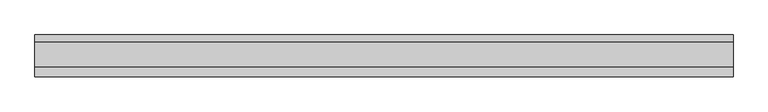
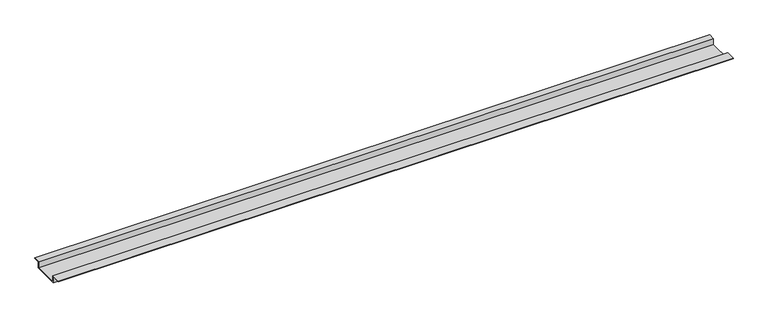
"""IFC4 building model written with IfcOpenShell, lengths in millimetres: proxy geometry, Soffit006 3743 : Soffit006 3743."""

from ifc_helpers import new_model, si_unit, frame, origin, place, context, project, spatial, polyline, outline, extrude, source, transform, mapped, element, save


def generic_models_bf3b7db1(model_context):
    return source(origin(), model_context, "Body", "SweptSolid", [
        extrude(outline(polyline([(10083.3424755, 39568.5010938), (10083.3424755, 39549.4130566), (10007.1424756, 39549.4130566), (10007.1424756, 39568.5072607), (9980.8881005, 39568.5072607), (9980.8881005, 39569.7771774), (10008.4125588, 39569.7771774), (10008.4125588, 39550.6830566), (10082.0724755, 39550.6830566), (10082.0724755, 39569.7710938), (10101.2017698, 39569.7710938), (10101.2017698, 39568.5010938), (10083.3424755, 39568.5010938)])), frame((3694.0383192, 0.0, 0.0), z_axis=(1.0, 0.0, 0.0), x_axis=(0.0, 1.0, 0.0)), (0.0, 0.0, 1.0), 2000.25),
    ])


if __name__ == "__main__":
    model = new_model("IFC4")
    model_context = context("Model", 3, world=origin())
    ifc_project = project(units=[si_unit("LENGTHUNIT", "METRE", prefix="MILLI")], contexts=[model_context])
    site = spatial("IfcSite", under=ifc_project)
    building = spatial("IfcBuilding", under=site)
    placement = place(None, origin())
    generic_models_shape = generic_models_bf3b7db1(model_context)
    element("IfcBuildingElementProxy", 1, Name="Soffit006 3743 : Soffit006 3743", ObjectType="Soffit006 3743 : Soffit006 3743", at=placement, inside=building, context=model_context, shape_type="MappedRepresentation", body=[
        mapped(generic_models_shape, transform((0.0, 0.0, 0.0), x_axis=(1.0, 0.0, 0.0), y_axis=(0.0, 1.0, 0.0), z_axis=(0.0, 0.0, 1.0))),
    ])
    save(model, "model.ifc")

# Revit data of these elements
# Type "Soffit006 3743 : Soffit006 3743"
#   NameOverride = "Soffit006"
# Element 1 (IfcBuildingElementProxy, "Soffit006 3743 : Soffit006 3743")
#   Materials on its faces: "16 GA. COPPER SOFFIT VENT - VERIFY W/ ARCHITECT ON LOCATION"
# Materials
#   "16 GA. COPPER SOFFIT VENT - VERIFY W/ ARCHITECT ON LOCATION": class "Unassigned", colour RGB 85 255 127, transparency 0
